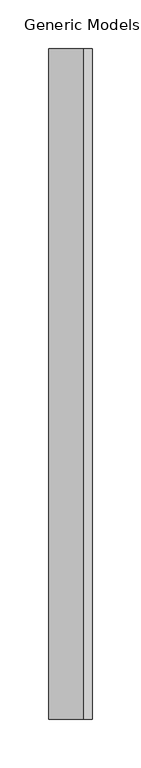
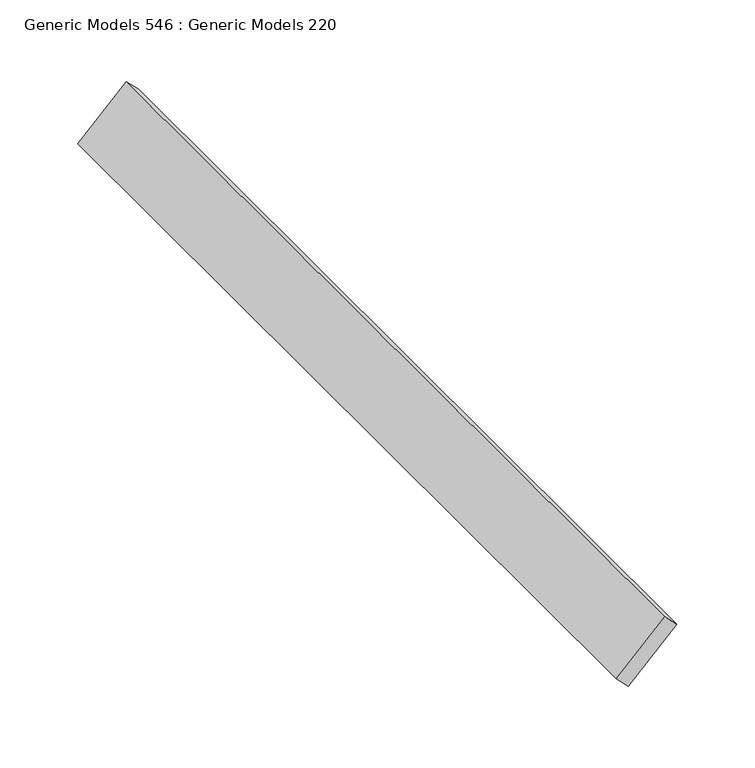
"""IFC4 building model written with IfcOpenShell, lengths in millimetres: proxy geometry, Generic Models 546 : Generic Models 220."""

from ifc_helpers import new_model, si_unit, frame, origin, place, context, project, spatial, polyline, outline, extrude, source, transform, mapped, element, save


def generic_models_546_generic_models_220_8a6de5d8(model_context):
    return source(origin(), model_context, "Body", "SweptSolid", [
        extrude(outline(polyline([(0.0, -12.7000001), (0.0, 0.0), (690.8142348, 0.0), (690.8142348, -12.7000001), (0.0, -12.7000001)])), frame((7841.3059863, 4539.4872686, 124811.1399101), z_axis=(0.7071067811868034, 0.0, 0.7071067811862918), x_axis=(0.0, -1.0, 0.0)), (0.0, 0.0, 1.0), 50.8),
    ])


if __name__ == "__main__":
    model = new_model("IFC4")
    model_context = context("Model", 3, world=origin())
    ifc_project = project(units=[si_unit("LENGTHUNIT", "METRE", prefix="MILLI")], contexts=[model_context])
    site = spatial("IfcSite", under=ifc_project)
    building = spatial("IfcBuilding", under=site)
    placement = place(None, origin())
    generic_models_546_generic_models_220_shape = generic_models_546_generic_models_220_8a6de5d8(model_context)
    element("IfcBuildingElementProxy", 1, Name="Generic Models 546 : Generic Models 220", ObjectType="Generic Models 546 : Generic Models 220", at=placement, inside=building, context=model_context, shape_type="MappedRepresentation", body=[
        mapped(generic_models_546_generic_models_220_shape, transform((0.0, 0.0, 0.0), x_axis=(1.0, 0.0, 0.0), y_axis=(0.0, 1.0, 0.0), z_axis=(0.0, 0.0, 1.0))),
    ])
    save(model, "model.ifc")

# Revit data of these elements
# Element 1 (IfcBuildingElementProxy, "Generic Models 546 : Generic Models 220")
#   Materials on its faces: "_WOOD TONE ALUMINUM EXTRUSION SLAT BY KNOTWOOD"
# Materials
#   "_WOOD TONE ALUMINUM EXTRUSION SLAT BY KNOTWOOD": class "Generic", colour RGB 177 130 114, transparency 0, Cost = 0
